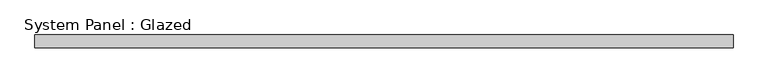
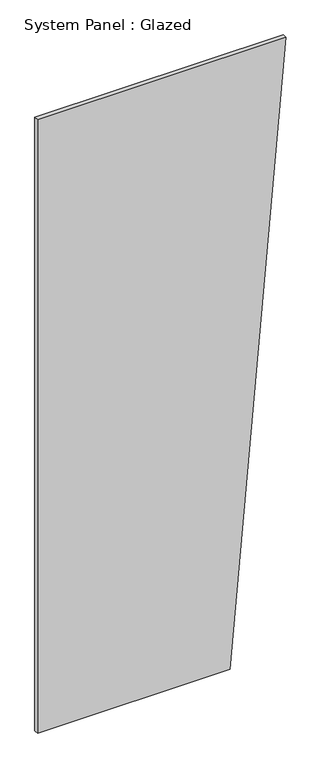
"""IFC4 building model written with IfcOpenShell, lengths in millimetres: plate geometry, System Panel : Glazed."""

from ifc_helpers import new_model, si_unit, frame, origin, place, context, project, spatial, polyline, outline, extrude, source, transform, mapped, element, save


def system_panel_glazed_b3fa7013(model_context):
    return source(origin(), model_context, "Body", "SweptSolid", [
        extrude(outline(polyline([(0.0, -701.3055584), (0.0, 386.1685195), (3657.6, 701.3055584), (3657.6, -701.3055584), (0.0, -701.3055584)])), frame((0.0, -44.45, 0.0), z_axis=(0.0, 1.0, 0.0), x_axis=(0.0, 0.0, 1.0)), (0.0, 0.0, 1.0), 25.4),
    ])


if __name__ == "__main__":
    model = new_model("IFC4")
    model_context = context("Model", 3, world=origin())
    ifc_project = project(units=[si_unit("LENGTHUNIT", "METRE", prefix="MILLI")], contexts=[model_context])
    site = spatial("IfcSite", under=ifc_project)
    building = spatial("IfcBuilding", under=site)
    placement = place(None, origin())
    system_panel_glazed_shape = system_panel_glazed_b3fa7013(model_context)
    element("IfcPlate", 1, ObjectType="System Panel : Glazed", at=placement, inside=building, context=model_context, shape_type="MappedRepresentation", body=[
        mapped(system_panel_glazed_shape, transform((0.0, 0.0, 0.0), x_axis=(1.0, 0.0, 0.0), y_axis=(0.0, 1.0, 0.0), z_axis=(0.0, 0.0, 1.0))),
    ])
    save(model, "model.ifc")

# Revit data of these elements
# Type "System Panel : Glazed"
#   Construction Type Id = "GSP4R"
#   Analytic Construction = "1/8 in Pilkington single glazing"
#   Visual Light Transmittance = 0.9
#   Solar Heat Gain Coefficient = 0.86
#   Heat Transfer Coefficient (U) = 1.18115 BTU/(h·ft²·°F)
#   Define Thermal Properties by = 1
# Element 1 (IfcPlate, "System Panel : Glazed")
#   Materials on its faces: "Glass"
# Materials
#   "Glass": class "Glass", colour RGB 0 128 192, transparency 0.75, Description = "Soda Lime Glass", Cost = 0
